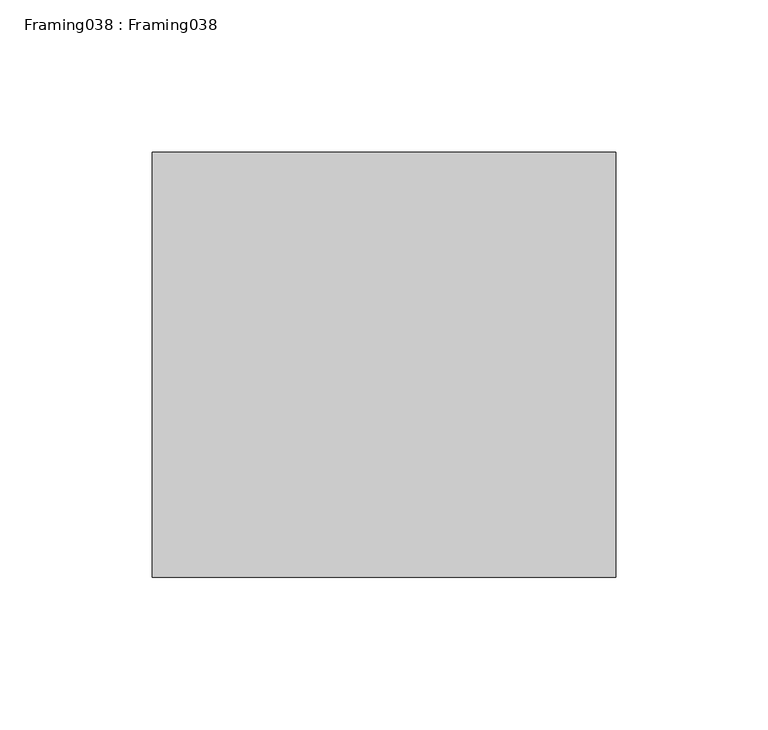
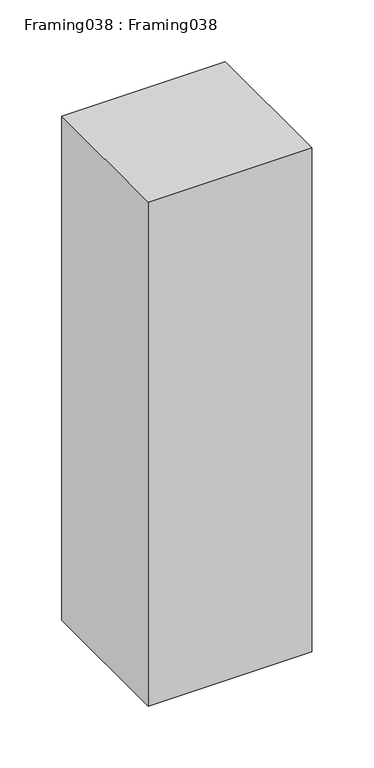
"""IFC4 building model written with IfcOpenShell, lengths in millimetres: proxy geometry, Framing038 : Framing038."""

from ifc_helpers import new_model, si_unit, frame, origin, place, context, project, spatial, polyline, outline, extrude, source, transform, mapped, element, save


def framing038_framing038_4d5a3201(model_context):
    return source(origin(), model_context, "Body", "SweptSolid", [
        extrude(outline(polyline([(12535.4175781, -4497.8424805), (12535.4175781, -4637.5424805), (12383.0175781, -4637.5424805), (12383.0175781, -4497.8424805), (12535.4175781, -4497.8424805)])), frame((0.0, 0.0, 39158.796875), z_axis=(0.0, 0.0, 1.0), x_axis=(1.0, 0.0, 0.0)), (0.0, 0.0, 1.0), 496.699125),
    ])


if __name__ == "__main__":
    model = new_model("IFC4")
    model_context = context("Model", 3, world=origin())
    ifc_project = project(units=[si_unit("LENGTHUNIT", "METRE", prefix="MILLI")], contexts=[model_context])
    site = spatial("IfcSite", under=ifc_project)
    building = spatial("IfcBuilding", under=site)
    placement = place(None, origin())
    framing038_framing038_shape = framing038_framing038_4d5a3201(model_context)
    element("IfcBuildingElementProxy", 1, Name="Framing038 : Framing038", ObjectType="Framing038 : Framing038", at=placement, inside=building, context=model_context, shape_type="MappedRepresentation", body=[
        mapped(framing038_framing038_shape, transform((0.0, 0.0, 0.0), x_axis=(1.0, 0.0, 0.0), y_axis=(0.0, 1.0, 0.0), z_axis=(0.0, 0.0, 1.0))),
    ])
    save(model, "model.ifc")

# Revit data of these elements
# Type "Framing038 : Framing038"
#   NameOverride = "Framing038"
# Element 1 (IfcBuildingElementProxy, "Framing038 : Framing038")
#   Materials on its faces: "WOOD FRAMING (SEE STRUCT DWGS)"
# Materials
#   "WOOD FRAMING (SEE STRUCT DWGS)": class "Unassigned", colour RGB 224 188 168, transparency 0, Cost = 0
